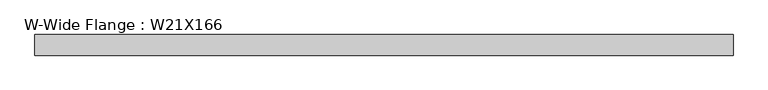
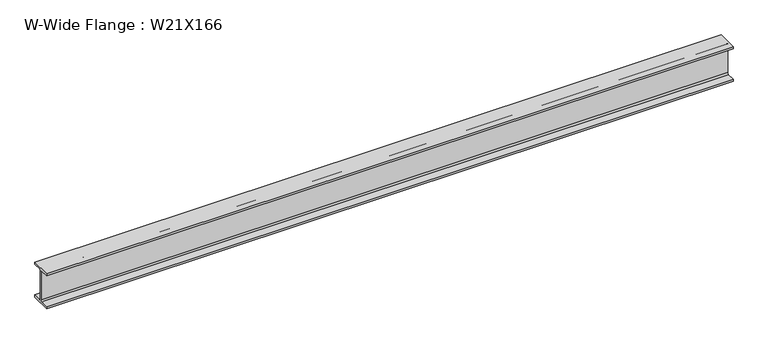
"""IFC4 building model written with IfcOpenShell, lengths in millimetres: beam geometry, W-Wide Flange : W21X166."""

from ifc_helpers import new_model, si_unit, point, frame, frame_2d, origin, place, context, project, spatial, polyline, circle_curve, trimmed, segment, composite_curve, outline, extrude, source, transform, mapped, element, save


def w_wide_flange_w21x166_04ac7672(model_context):
    return source(origin(), model_context, "Body", "SweptSolid", [
        extrude(outline(composite_curve([segment(polyline([(157.48, -251.206), (157.48, -285.75), (-157.48, -285.75), (-157.48, -251.206), (-32.131, -251.206)]), True, "CONTINUOUS"), segment(trimmed(circle_curve(frame_2d((-32.131, -228.6)), 22.606), [point((-32.131, -251.206))], [point((-9.525, -228.6))], True, "CARTESIAN"), True, "CONTINUOUS"), segment(polyline([(-9.525, -228.6), (-9.525, 228.6)]), True, "CONTINUOUS"), segment(trimmed(circle_curve(frame_2d((-32.131, 228.6)), 22.606), [point((-9.525, 228.6))], [point((-32.131, 251.206))], True, "CARTESIAN"), True, "CONTINUOUS"), segment(polyline([(-32.131, 251.206), (-157.48, 251.206), (-157.48, 285.75), (157.48, 285.75), (157.48, 251.206), (32.131, 251.206)]), True, "CONTINUOUS"), segment(trimmed(circle_curve(frame_2d((32.131, 228.6)), 22.606), [point((32.131, 251.206))], [point((9.525, 228.6))], True, "CARTESIAN"), True, "CONTINUOUS"), segment(polyline([(9.525, 228.6), (9.525, -228.6)]), True, "CONTINUOUS"), segment(trimmed(circle_curve(frame_2d((32.131, -228.6)), 22.606), [point((9.525, -228.6))], [point((32.131, -251.206))], True, "CARTESIAN"), True, "CONTINUOUS"), segment(polyline([(32.131, -251.206), (157.48, -251.206)]), True, "CONTINUOUS")], self_intersect=False)), frame((-5429.1838829, 0.0, 0.0), z_axis=(1.0, 0.0, 0.0), x_axis=(0.0, 1.0, 0.0)), (0.0, 0.0, 1.0), 10659.8214497),
    ])


if __name__ == "__main__":
    model = new_model("IFC4")
    model_context = context("Model", 3, world=origin())
    ifc_project = project(units=[si_unit("LENGTHUNIT", "METRE", prefix="MILLI")], contexts=[model_context])
    site = spatial("IfcSite", under=ifc_project)
    building = spatial("IfcBuilding", under=site)
    placement = place(None, origin())
    w_wide_flange_w21x166_shape = w_wide_flange_w21x166_04ac7672(model_context)
    element("IfcBeam", 1, ObjectType="W-Wide Flange : W21X166", at=placement, inside=building, context=model_context, shape_type="MappedRepresentation", body=[
        mapped(w_wide_flange_w21x166_shape, transform((0.0, 0.0, 0.0), x_axis=(1.0, 0.0, 0.0), y_axis=(0.0, 1.0, 0.0), z_axis=(0.0, 0.0, 1.0))),
    ])
    save(model, "model.ifc")

# Revit data of these elements
# Type "W-Wide Flange : W21X166"
#   Assembly Code = "B10"
#   W = 166
#   Length [instance default] = 5' - 0"
#   bf = 1' - 0.4"
#   d = 1' - 10 1/2"
#   k = 0' - 2 1/4"
#   k2 = 0' - 0.89"
#   tf = 0' - 1.36"
#   tw = 0' - 0 3/4"
#   A = 0.338889 SF
#   Structural Material [instance default] = Steel ASTM A992
# Element 1 (IfcBeam, "W-Wide Flange : W21X166")
#   Structural Material = Steel
#   Materials on its faces: "Steel"
# Materials
#   "Steel ASTM A992": class "Metal", colour RGB 199 199 199, transparency 0, Description = "Structural steel 50ksi", Cost = 0
#   "Steel": class "Metal", colour RGB 118 118 114, transparency 0, Description = "Steel, mill finish", Cost = 0
